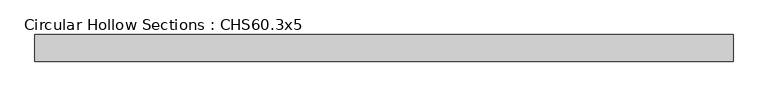
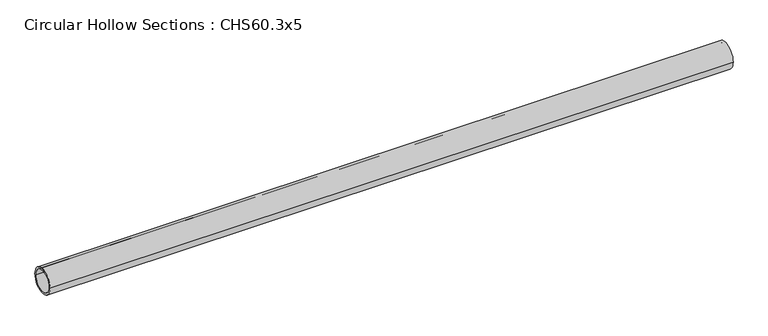
"""IFC4 building model written with IfcOpenShell, lengths in millimetres: beam geometry, Circular Hollow Sections : CHS60.3x5."""

import ifcopenshell
import ifcopenshell.guid

model = None  # the IFC model being written
_history = None  # IfcOwnerHistory: only IFC2X3 demands one
_inside = {}  # id of a spatial element -> (the spatial element, [elements in it])
_under = {}  # id of a project, library or spatial element -> (it, [spatial elements below it])
_declared = {}  # id of a project -> (the project, [libraries it declares])
_typed = {}  # id of a type object -> (the type object, [elements of that type])
_made_of = {}  # id of a material, layer set ... -> (it, [elements and type objects made of it])


def new_model(schema):
    """Start an empty IFC model of exactly this schema.

    Asked for "IFC4X3", IfcOpenShell would pick the latest addendum, in which some entities
    have other attributes; the version numbers below select the first issue.
    IFC2X3 requires an IfcOwnerHistory on every rooted entity: one is made here for all.
    """
    global model, _history
    if schema == "IFC4X3":
        model = ifcopenshell.file(schema_version=(4, 3, 0, 0))
    else:
        model = ifcopenshell.file(schema=schema)
    _inside.clear()
    _under.clear()
    _declared.clear()
    _typed.clear()
    _made_of.clear()
    _history = None
    if model.schema == "IFC2X3":
        org = make("IfcOrganization", Name="unknown")
        user = make(
            "IfcPersonAndOrganization",
            ThePerson=make("IfcPerson", FamilyName="unknown"),
            TheOrganization=org,
        )
        app = make(
            "IfcApplication",
            ApplicationDeveloper=org,
            Version="unknown",
            ApplicationFullName="unknown",
            ApplicationIdentifier="unknown",
        )
        _history = make(
            "IfcOwnerHistory",
            OwningUser=user,
            OwningApplication=app,
            ChangeAction="ADDED",
            CreationDate=0,
        )
    return model


def make(cls, **values):
    """One entity of the class cls with the attributes given. An attribute that is None is left unset."""
    return model.create_entity(
        cls, **{name: value for name, value in values.items() if value is not None}
    )


def rooted(cls, **values):
    """An entity with a GlobalId (a new one), such as an element, a storey or a relation."""
    return make(cls, GlobalId=ifcopenshell.guid.new(), OwnerHistory=_history, **values)


def si_unit(unit_type, name, prefix=None):
    """IfcSIUnit, for example si_unit("LENGTHUNIT", "METRE", prefix="MILLI")."""
    return make("IfcSIUnit", UnitType=unit_type, Prefix=prefix, Name=name)


def assignment(units):
    """IfcUnitAssignment: the units of a project."""
    return None if units is None else make("IfcUnitAssignment", Units=units)


def point(xyz):
    """IfcCartesianPoint."""
    return None if xyz is None else make("IfcCartesianPoint", Coordinates=xyz)


def direction(xyz):
    """IfcDirection."""
    return None if xyz is None else make("IfcDirection", DirectionRatios=xyz)


def frame(location, z_axis=None, x_axis=None):
    """IfcAxis2Placement3D, a coordinate frame: its origin and axes. An axis left out is left unset."""
    return make(
        "IfcAxis2Placement3D",
        Location=point(location),
        Axis=direction(z_axis),
        RefDirection=direction(x_axis),
    )


def frame_2d(location, x_axis=None):
    """IfcAxis2Placement2D, a coordinate frame in the plane: its origin and x axis."""
    return make(
        "IfcAxis2Placement2D", Location=point(location), RefDirection=direction(x_axis)
    )


def origin():
    """The frame at (0, 0, 0) with its axes left unset."""
    return frame((0.0, 0.0, 0.0))


def origin_2d():
    """The frame at (0, 0) in the plane with its x axis left unset."""
    return frame_2d((0.0, 0.0))


def place(relative_to, where):
    """IfcLocalPlacement: puts the frame where relative to a parent placement (None: the world)."""
    return make(
        "IfcLocalPlacement", PlacementRelTo=relative_to, RelativePlacement=where
    )


def context(
    kind, dimensions, precision=None, world=None, true_north=None, identifier=None
):
    """IfcGeometricRepresentationContext, for example the 3D "Model" context."""
    return make(
        "IfcGeometricRepresentationContext",
        ContextIdentifier=identifier,
        ContextType=kind,
        CoordinateSpaceDimension=dimensions,
        Precision=precision,
        WorldCoordinateSystem=world,
        TrueNorth=true_north,
    )


def project(units=None, contexts=None):
    """IfcProject with its units and contexts."""
    return rooted(
        "IfcProject",
        Name="project",
        RepresentationContexts=contexts,
        UnitsInContext=assignment(units),
    )


def spatial(cls, under=None, at=None, **own):
    """A site, building, storey or space (cls), placed at a placement, below another one or the project."""
    s = rooted(cls, ObjectPlacement=at, **own)
    if under is not None:
        _under.setdefault(under.id(), (under, []))[1].append(s)
    return s


def circle_curve(where, radius):
    """IfcCircle in the frame where."""
    return make("IfcCircle", Position=where, Radius=radius)


def trimmed(basis, trim1, trim2, sense, master):
    """IfcTrimmedCurve: the piece of a basis curve between two trims."""
    return make(
        "IfcTrimmedCurve",
        BasisCurve=basis,
        Trim1=trim1,
        Trim2=trim2,
        SenseAgreement=sense,
        MasterRepresentation=master,
    )


def segment(curve, same_sense, transition):
    """IfcCompositeCurveSegment."""
    return make(
        "IfcCompositeCurveSegment",
        Transition=transition,
        SameSense=same_sense,
        ParentCurve=curve,
    )


def composite_curve(segments, self_intersect=None):
    """IfcCompositeCurve: segments joined end to end."""
    return make("IfcCompositeCurve", Segments=segments, SelfIntersect=self_intersect)


def outline(outer, holes=None, kind="AREA"):
    """IfcArbitraryClosedProfileDef: a profile drawn as a closed curve; with holes, ...WithVoids."""
    if holes is None:
        return make("IfcArbitraryClosedProfileDef", ProfileType=kind, OuterCurve=outer)
    return make(
        "IfcArbitraryProfileDefWithVoids",
        ProfileType=kind,
        OuterCurve=outer,
        InnerCurves=holes,
    )


def extrude(swept, where, along, depth):
    """IfcExtrudedAreaSolid: the profile swept, set in the frame where, extruded along a direction by depth."""
    return make(
        "IfcExtrudedAreaSolid",
        SweptArea=swept,
        Position=where,
        ExtrudedDirection=direction(along),
        Depth=depth,
    )


def shape(context_of_items, identifier, shape_type, items):
    """IfcShapeRepresentation: the items that make up one representation, for example the "Body"."""
    return make(
        "IfcShapeRepresentation",
        ContextOfItems=context_of_items,
        RepresentationIdentifier=identifier,
        RepresentationType=shape_type,
        Items=items,
    )


def source(mapping_origin, context_of_items, identifier, shape_type, items):
    """IfcRepresentationMap: a shape defined once, which mapped items show again and again."""
    return make(
        "IfcRepresentationMap",
        MappingOrigin=mapping_origin,
        MappedRepresentation=shape(context_of_items, identifier, shape_type, items),
    )


def transform(
    local_origin,
    x_axis=None,
    y_axis=None,
    z_axis=None,
    scale=None,
    scale2=None,
    scale3=None,
    uniform=True,
):
    """IfcCartesianTransformationOperator3D, or its non-uniform kind. x_axis, y_axis, z_axis: its Axis1, 2, 3."""
    if uniform:
        return make(
            "IfcCartesianTransformationOperator3D",
            Axis1=direction(x_axis),
            Axis2=direction(y_axis),
            LocalOrigin=point(local_origin),
            Scale=scale,
            Axis3=direction(z_axis),
        )
    return make(
        "IfcCartesianTransformationOperator3DnonUniform",
        Axis1=direction(x_axis),
        Axis2=direction(y_axis),
        LocalOrigin=point(local_origin),
        Scale=scale,
        Axis3=direction(z_axis),
        Scale2=scale2,
        Scale3=scale3,
    )


def mapped(mapping_source, mapping_target):
    """IfcMappedItem: shows the shape of a source again, moved by a transform."""
    return make(
        "IfcMappedItem", MappingSource=mapping_source, MappingTarget=mapping_target
    )


def made_of(thing, what):
    """Note that an element or type object is made of a material, layer set ...; save() writes the relation."""
    if what is not None:
        _made_of.setdefault(what.id(), (what, []))[1].append(thing)
    return thing


def element(
    cls,
    number,
    at=None,
    inside=None,
    cuts=None,
    type_object=None,
    material=None,
    context=None,
    identifier="Body",
    shape_type=None,
    held_by="IfcProductDefinitionShape",
    body=None,
    shapes=None,
    **own,
):
    """One element of the class cls, such as IfcWall. Its Tag is "e" and its number.

    at: its placement. inside: the storey or other place that contains it. cuts: it is an
    opening in that element (IfcRelVoidsElement). A single representation is given by context,
    identifier, shape_type and body (its items); several are given by shapes. held_by: the class
    of the entity that holds the representations. save() writes the other relations.
    """
    e = rooted(cls, Tag="e%d" % number, ObjectPlacement=at, **own)
    if body is not None:
        shapes = [shape(context, identifier, shape_type, body)]
    if shapes is not None:
        e.Representation = make(held_by, Representations=shapes)
    if inside is not None:
        _inside.setdefault(inside.id(), (inside, []))[1].append(e)
    if cuts is not None:
        rooted(
            "IfcRelVoidsElement", RelatingBuildingElement=cuts, RelatedOpeningElement=e
        )
    if type_object is not None:
        _typed.setdefault(type_object.id(), (type_object, []))[1].append(e)
    return made_of(e, material)


def aggregate(whole, parts):
    """IfcRelAggregates: a whole, such as a stair, and the parts it consists of."""
    return rooted("IfcRelAggregates", RelatingObject=whole, RelatedObjects=parts)


def save(model, path):
    """Write the relations noted so far, then the file.

    IfcRelAggregates (storeys below a building ...), IfcRelContainedInSpatialStructure (elements
    in a storey), IfcRelDefinesByType, IfcRelAssociatesMaterial and IfcRelDeclares: one each for
    every whole, place, type object, material and project.
    """
    for whole, parts in _under.values():
        aggregate(whole, parts)
    for where, things in _inside.values():
        rooted(
            "IfcRelContainedInSpatialStructure",
            RelatedElements=things,
            RelatingStructure=where,
        )
    for kind, things in _typed.values():
        rooted("IfcRelDefinesByType", RelatedObjects=things, RelatingType=kind)
    for what, things in _made_of.values():
        rooted("IfcRelAssociatesMaterial", RelatedObjects=things, RelatingMaterial=what)
    for by, libraries in _declared.values():
        rooted("IfcRelDeclares", RelatingContext=by, RelatedDefinitions=libraries)
    model.write(path)


def circular_hollow_sections_chs60_3x5_b8a643cb(model_context):
    return source(origin(), model_context, "Body", "SweptSolid", [
        extrude(outline(composite_curve([segment(trimmed(circle_curve(origin_2d(), 30.15), [point((-30.15, 0.0))], [point((30.15, 0.0))], False, "CARTESIAN"), True, "CONTINUOUS"), segment(trimmed(circle_curve(origin_2d(), 30.15), [point((30.15, 0.0))], [point((-30.15, 0.0))], False, "CARTESIAN"), True, "CONTINUOUS")], self_intersect=False), holes=[composite_curve([segment(trimmed(circle_curve(origin_2d(), 25.15), [point((25.15, 0.0))], [point((-25.15, 0.0))], True, "CARTESIAN"), True, "CONTINUOUS"), segment(trimmed(circle_curve(origin_2d(), 25.15), [point((-25.15, 0.0))], [point((25.15, 0.0))], True, "CARTESIAN"), True, "CONTINUOUS")], self_intersect=False)]), frame((-790.0, 0.0, 0.0), z_axis=(1.0, 0.0, 0.0), x_axis=(0.0, 1.0, 0.0)), (0.0, 0.0, 1.0), 1580.0),
    ])


if __name__ == "__main__":
    model = new_model("IFC4")
    model_context = context("Model", 3, world=origin())
    ifc_project = project(units=[si_unit("LENGTHUNIT", "METRE", prefix="MILLI")], contexts=[model_context])
    site = spatial("IfcSite", under=ifc_project)
    building = spatial("IfcBuilding", under=site)
    placement = place(None, origin())
    circular_hollow_sections_chs60_3x5_shape = circular_hollow_sections_chs60_3x5_b8a643cb(model_context)
    element("IfcBeam", 1, ObjectType="Circular Hollow Sections : CHS60.3x5", at=placement, inside=building, context=model_context, shape_type="MappedRepresentation", body=[
        mapped(circular_hollow_sections_chs60_3x5_shape, transform((0.0, 0.0, 0.0), x_axis=(1.0, 0.0, 0.0), y_axis=(0.0, 1.0, 0.0), z_axis=(0.0, 0.0, 1.0))),
    ])
    save(model, "model.ifc")

# Revit data of these elements
# Type "Circular Hollow Sections : CHS60.3x5"
#   Description = "Hollow Core Steel Roof Truss Member"
#   Type Comments = "Steel 50-355"
#   Assembly Code = "F10"
#   t = 5 mm
#   W = 0.00682
#   Start Extension Calculation [instance default] = 3000 mm
#   Start Extension [instance default] = -12.7 mm
#   Length [instance default] = 1500 mm
#   OD = 60.3 mm
#   End Extension Calculation [instance default] = 3000 mm
#   End Extension [instance default] = -12.7 mm
#   A = 0.000869 m²
#   Structural Material [instance default] = Metal - Steel 50-355
# Element 1 (IfcBeam, "Circular Hollow Sections : CHS60.3x5")
#   Materials on its faces: "Metal - Steel 50-355"
# Materials
#   "Metal - Steel 50-355": class "Metal", colour RGB 247 247 247, transparency 0
